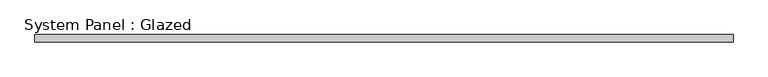
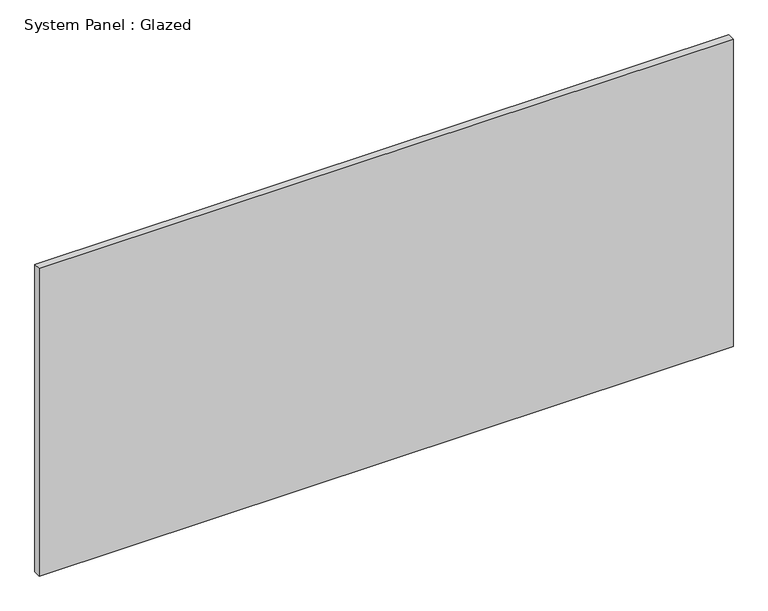
"""IFC4 building model written with IfcOpenShell, lengths in millimetres: plate geometry, System Panel : Glazed."""

from ifc_helpers import new_model, si_unit, origin, origin_with_axes, place, context, project, spatial, polyline, outline, extrude, source, transform, mapped, element, save


def system_panel_glazed_5b1e694d(model_context):
    return source(origin(), model_context, "Body", "SweptSolid", [
        extrude(outline(polyline([(1199.1815359, -44.45), (-1199.1815359, -44.45), (-1199.1815359, -19.05), (1199.1815359, -19.05), (1199.1815359, -44.45)])), origin_with_axes(), (0.0, 0.0, 1.0), 1123.95),
    ])


if __name__ == "__main__":
    model = new_model("IFC4")
    model_context = context("Model", 3, world=origin())
    ifc_project = project(units=[si_unit("LENGTHUNIT", "METRE", prefix="MILLI")], contexts=[model_context])
    site = spatial("IfcSite", under=ifc_project)
    building = spatial("IfcBuilding", under=site)
    placement = place(None, origin())
    system_panel_glazed_shape = system_panel_glazed_5b1e694d(model_context)
    element("IfcPlate", 1, ObjectType="System Panel : Glazed", at=placement, inside=building, context=model_context, shape_type="MappedRepresentation", body=[
        mapped(system_panel_glazed_shape, transform((0.0, 0.0, 0.0), x_axis=(1.0, 0.0, 0.0), y_axis=(0.0, 1.0, 0.0), z_axis=(0.0, 0.0, 1.0))),
    ])
    save(model, "model.ifc")

# Revit data of these elements
# Type "System Panel : Glazed"
#   Construction Type Id = "GSP4R"
#   Analytic Construction = "1/8 in Pilkington single glazing"
#   Visual Light Transmittance = 0.9
#   Solar Heat Gain Coefficient = 0.86
#   Heat Transfer Coefficient (U) = 1.18115 BTU/(h·ft²·°F)
#   Define Thermal Properties by = 1
# Element 1 (IfcPlate, "System Panel : Glazed")
#   Materials on its faces: "Glass"
# Materials
#   "Glass": class "Glass", colour RGB 0 128 192, transparency 0.75, Description = "Soda Lime Glass", Cost = 0
